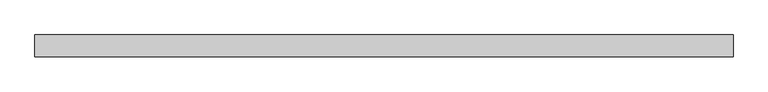
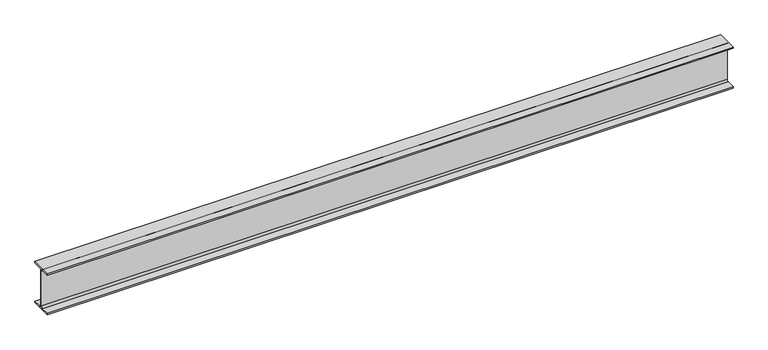
"""IFC4 building model written with IfcOpenShell, lengths in millimetres: beam geometry, 0912_Steel Framing_H-KSD3502 : H_SB_AR_S02_H-300x150x6.5x9_Stair."""

from ifc_helpers import new_model, si_unit, point, frame, frame_2d, origin, place, context, project, spatial, polyline, circle_curve, trimmed, segment, composite_curve, outline, extrude, source, transform, mapped, element, save


def beam_a4a24592(model_context):
    return source(origin(), model_context, "Body", "SweptSolid", [
        extrude(outline(composite_curve([segment(polyline([(75.0, -141.0), (75.0, -150.0), (-75.0, -150.0), (-75.0, -141.0), (-16.25, -141.0)]), True, "CONTINUOUS"), segment(trimmed(circle_curve(frame_2d((-16.25, -128.0)), 13.0), [point((-16.25, -141.0))], [point((-3.25, -128.0))], True, "CARTESIAN"), True, "CONTINUOUS"), segment(polyline([(-3.25, -128.0), (-3.25, 128.0)]), True, "CONTINUOUS"), segment(trimmed(circle_curve(frame_2d((-16.25, 128.0)), 13.0), [point((-3.25, 128.0))], [point((-16.25, 141.0))], True, "CARTESIAN"), True, "CONTINUOUS"), segment(polyline([(-16.25, 141.0), (-75.0, 141.0), (-75.0, 150.0), (75.0, 150.0), (75.0, 141.0), (16.25, 141.0)]), True, "CONTINUOUS"), segment(trimmed(circle_curve(frame_2d((16.25, 128.0)), 13.0), [point((16.25, 141.0))], [point((3.25, 128.0))], True, "CARTESIAN"), True, "CONTINUOUS"), segment(polyline([(3.25, 128.0), (3.25, -128.0)]), True, "CONTINUOUS"), segment(trimmed(circle_curve(frame_2d((16.25, -128.0)), 13.0), [point((3.25, -128.0))], [point((16.25, -141.0))], True, "CARTESIAN"), True, "CONTINUOUS"), segment(polyline([(16.25, -141.0), (75.0, -141.0)]), True, "CONTINUOUS")], self_intersect=False)), frame((-2387.3, 0.0, 0.0), z_axis=(1.0, 0.0, 0.0), x_axis=(0.0, 1.0, 0.0)), (0.0, 0.0, 1.0), 4774.6),
    ])


if __name__ == "__main__":
    model = new_model("IFC4")
    model_context = context("Model", 3, world=origin())
    ifc_project = project(units=[si_unit("LENGTHUNIT", "METRE", prefix="MILLI")], contexts=[model_context])
    site = spatial("IfcSite", under=ifc_project)
    building = spatial("IfcBuilding", under=site)
    placement = place(None, origin())
    beam_shape = beam_a4a24592(model_context)
    element("IfcBeam", 1, ObjectType="0912_Steel Framing_H-KSD3502 : H_SB_AR_S02_H-300x150x6.5x9_Stair", at=placement, inside=building, context=model_context, shape_type="MappedRepresentation", body=[
        mapped(beam_shape, transform((0.0, 0.0, 0.0), x_axis=(1.0, 0.0, 0.0), y_axis=(0.0, 1.0, 0.0), z_axis=(0.0, 0.0, 1.0))),
    ])
    save(model, "model.ifc")

# Revit data of these elements
# Type "0912_Steel Framing_H-KSD3502 : H_SB_AR_S02_H-300x150x6.5x9_Stair"
#   H_Q'ty Cal Type Tag = "SB-Q2"
#   H_WM Code_1 = "S01AA073-00001 |  | TON | Main Steel Structure Fabrication Work | Shelter/Building | Medium Steel - Standard |  |  |  |  |  |  | Material: (   ) | (90)KG/M>Weight≥(30)KG/M | S01AA073-00001 Main Steel Structure Fabrication Work Shelter/Building Medium Steel - Standard         | - Material: ( ASTM A36 )\n- (90)KG/M>Weight≥(30)KG/M"
#   H_WM Code_2 = "S03AA083-00001 |  | TON | Main Steel Structure Erection Work | Shelter/Building | Medium Steel |  |  |  |  |  |  | Material: (   ) | S03AA083-00001 Main Steel Structure Erection Work Shelter/Building Medium Steel         | - Material: ( ASTM A36 )"
#   H_WM Code_3 = "S01AA009-00001 |  | TON | Main Steel Structure Fabrication Work | Shelter/Building | Plates - Gusset, Stiffener, ETC | Material: (   ) | S01AA009-00001 Main Steel Structure Fabrication Work Shelter/Building Plates - Gusset, Stiffener, ETC         |"
#   H_WM Code_4 = "S41AA051-00001 |  | M2 | Steel Structure Paint Work | Shelter/Building | for Non-Fireproofed Steel Surface |  |  |  |  |  |  | Material: (   ) | S41AA051-00001 Steel Structure Paint Work Shelter/Building for Non-Fireproofed Steel Surface         |"
#   Width = 15.0 cm
#   Web Thickness = 0.65 cm
#   Web Fillet = 1.3 cm
#   Warping Constant = 107000.0 cm⁶
#   W = 0
#   Torsional Moment of Inertia = 9.9539 cm⁴
#   Section Area = 46.78 cm²
#   Plastic Modulus weak axis = 105.0 cm³
#   Plastic Modulus strong axis = 542.0 cm³
#   Perimeter = 1.17 m²/m
#   Nominal Weight = 36.70 kgf/m
#   Moment of Inertia weak axis = 508.00 cm⁴
#   Moment of Inertia strong axis = 7210.00 cm⁴
#   Height = 30.0 cm
#   Flange Thickness = 0.9 cm
#   Elastic Modulus weak axis = 67.7 cm³
#   Elastic Modulus strong axis = 481.0 cm³
#   Centroid Vertical = 15.0 cm
#   Centroid Horizontal = 7.5 cm
#   Ix = 72100000
#   Length [instance default] = 1524 mm
#   Zx = 542000
#   b = 150 mm
#   h = 300 mm
#   r = 13 mm
#   s = 6.5 mm
#   t = 9 mm
#   A = 0.004678 m²
#   Structural Material [instance default] = Steel, 45-345
#   Assembly Code = ""
# Element 1 (IfcBeam, "0912_Steel Framing_H-KSD3502 : H_SB_AR_S02_H-300x150x6.5x9_Stair")
#   Materials on its faces: "Steel, 45-345"
# Materials
#   "Steel, 45-345": class "Metal", colour RGB 189 187 185, transparency 0, Description = "Steel 345 MPa", Cost = 0
